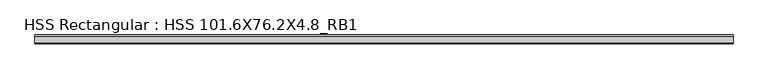
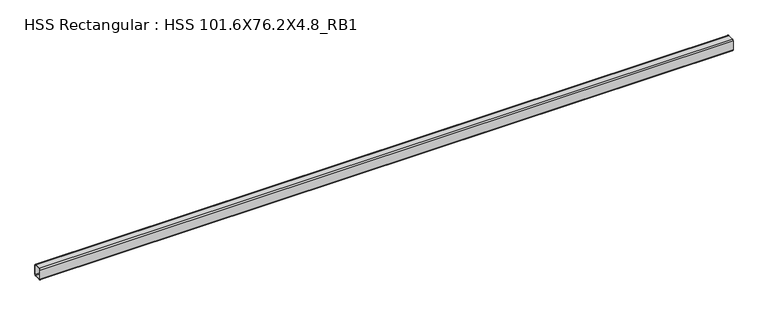
"""IFC4 building model written with IfcOpenShell, lengths in millimetres: beam geometry, HSS Rectangular : HSS 101.6X76.2X4.8_RB1."""

from ifc_helpers import new_model, si_unit, point, frame, frame_2d, origin, place, context, project, spatial, polyline, circle_curve, trimmed, segment, composite_curve, outline, extrude, source, transform, mapped, element, save


def hss_rectangular_hss_101_6x76_2x4_8_rb1_88f4fb49(model_context):
    return source(origin(), model_context, "Body", "SweptSolid", [
        extrude(outline(composite_curve([segment(polyline([(38.1, 41.275), (38.1, -41.275)]), True, "CONTINUOUS"), segment(trimmed(circle_curve(frame_2d((28.575, -41.275)), 9.525), [point((38.1, -41.275))], [point((28.575, -50.8))], False, "CARTESIAN"), True, "CONTINUOUS"), segment(polyline([(28.575, -50.8), (-28.575, -50.8)]), True, "CONTINUOUS"), segment(trimmed(circle_curve(frame_2d((-28.575, -41.275)), 9.525), [point((-28.575, -50.8))], [point((-38.1, -41.275))], False, "CARTESIAN"), True, "CONTINUOUS"), segment(polyline([(-38.1, -41.275), (-38.1, 41.275)]), True, "CONTINUOUS"), segment(trimmed(circle_curve(frame_2d((-28.575, 41.275)), 9.525), [point((-38.1, 41.275))], [point((-28.575, 50.8))], False, "CARTESIAN"), True, "CONTINUOUS"), segment(polyline([(-28.575, 50.8), (28.575, 50.8)]), True, "CONTINUOUS"), segment(trimmed(circle_curve(frame_2d((28.575, 41.275)), 9.525), [point((28.575, 50.8))], [point((38.1, 41.275))], False, "CARTESIAN"), True, "CONTINUOUS")], self_intersect=False), holes=[composite_curve([segment(trimmed(circle_curve(frame_2d((-28.575, 41.275)), 4.7625), [point((-28.575, 46.0375))], [point((-33.3375, 41.275))], True, "CARTESIAN"), True, "CONTINUOUS"), segment(polyline([(-33.3375, 41.275), (-33.3375, -41.275)]), True, "CONTINUOUS"), segment(trimmed(circle_curve(frame_2d((-28.575, -41.275)), 4.7625), [point((-33.3375, -41.275))], [point((-28.575, -46.0375))], True, "CARTESIAN"), True, "CONTINUOUS"), segment(polyline([(-28.575, -46.0375), (28.575, -46.0375)]), True, "CONTINUOUS"), segment(trimmed(circle_curve(frame_2d((28.575, -41.275)), 4.7625), [point((28.575, -46.0375))], [point((33.3375, -41.275))], True, "CARTESIAN"), True, "CONTINUOUS"), segment(polyline([(33.3375, -41.275), (33.3375, 41.275)]), True, "CONTINUOUS"), segment(trimmed(circle_curve(frame_2d((28.575, 41.275)), 4.7625), [point((33.3375, 41.275))], [point((28.575, 46.0375))], True, "CARTESIAN"), True, "CONTINUOUS"), segment(polyline([(28.575, 46.0375), (-28.575, 46.0375)]), True, "CONTINUOUS")], self_intersect=False)]), frame((-7525.9966117, 0.0, 0.0), z_axis=(1.0, 0.0, 0.0), x_axis=(0.0, 1.0, 0.0)), (0.0, 0.0, 1.0), 6013.0479004),
    ])


if __name__ == "__main__":
    model = new_model("IFC4")
    model_context = context("Model", 3, world=origin())
    ifc_project = project(units=[si_unit("LENGTHUNIT", "METRE", prefix="MILLI")], contexts=[model_context])
    site = spatial("IfcSite", under=ifc_project)
    building = spatial("IfcBuilding", under=site)
    placement = place(None, origin())
    hss_rectangular_hss_101_6x76_2x4_8_rb1_shape = hss_rectangular_hss_101_6x76_2x4_8_rb1_88f4fb49(model_context)
    element("IfcBeam", 1, ObjectType="HSS Rectangular : HSS 101.6X76.2X4.8_RB1", at=placement, inside=building, context=model_context, shape_type="MappedRepresentation", body=[
        mapped(hss_rectangular_hss_101_6x76_2x4_8_rb1_shape, transform((0.0, 0.0, 0.0), x_axis=(1.0, 0.0, 0.0), y_axis=(0.0, 1.0, 0.0), z_axis=(0.0, 0.0, 1.0))),
    ])
    save(model, "model.ifc")

# Revit data of these elements
# Type "HSS Rectangular : HSS 101.6X76.2X4.8_RB1"
#   Section Name Key = "HSS 4X3X3/16"
#   Assembly Code = "B10"
#   Width = 7.62 cm
#   Wall Nominal Thickness = 0.4763 cm
#   Wall Design Thickness = 0.442 cm
#   Torsional Moment of Inertia = 260.561 cm⁴
#   Torsional Modulus = 61.2876 cm³
#   Section Area = 14.4516 cm²
#   Plastic Modulus weak axis = 40.3122 cm³
#   Plastic Modulus strong axis = 49.1612 cm³
#   Perimeter = 0.881482 m²/m
#   Outer Fillet = 0.9525 cm
#   Nominal Weight = 12.1285 kgf/m
#   Moment of Inertia weak axis = 131.529 cm⁴
#   Moment of Inertia strong axis = 205.202 cm⁴
#   Inner Fillet = 0.4763 cm
#   Height = 10.16 cm
#   Elastic Modulus weak axis = 34.4128 cm³
#   Elastic Modulus strong axis = 40.476 cm³
#   Centroid Vertical = 5.08 cm
#   Centroid Horizontal = 3.81 cm
#   Length [instance default] = 1524 mm
#   Structural Material [instance default] = Steel ASTM A500, Grade B, Rectangular and Square
#   Principal Axes Angle = 0
# Element 1 (IfcBeam, "HSS Rectangular : HSS 101.6X76.2X4.8_RB1")
#   Structural Material = Steel ASTM A992
#   Materials on its faces: "Steel ASTM A992"
# Materials
#   "Steel ASTM A500, Grade B, Rectangular and Square": class "Metal", colour RGB 199 199 199, transparency 0, Description = "Carbon steel", Cost = 0
#   "Steel ASTM A992": class "Metal", colour RGB 199 199 199, transparency 0, Description = "Structural steel 50ksi", Cost = 0
